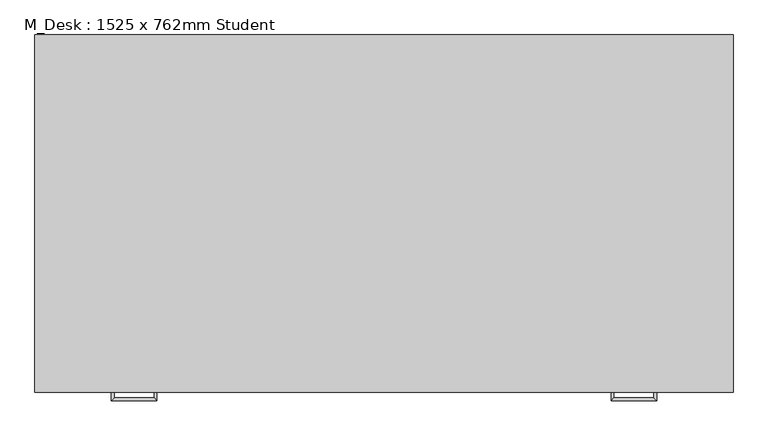
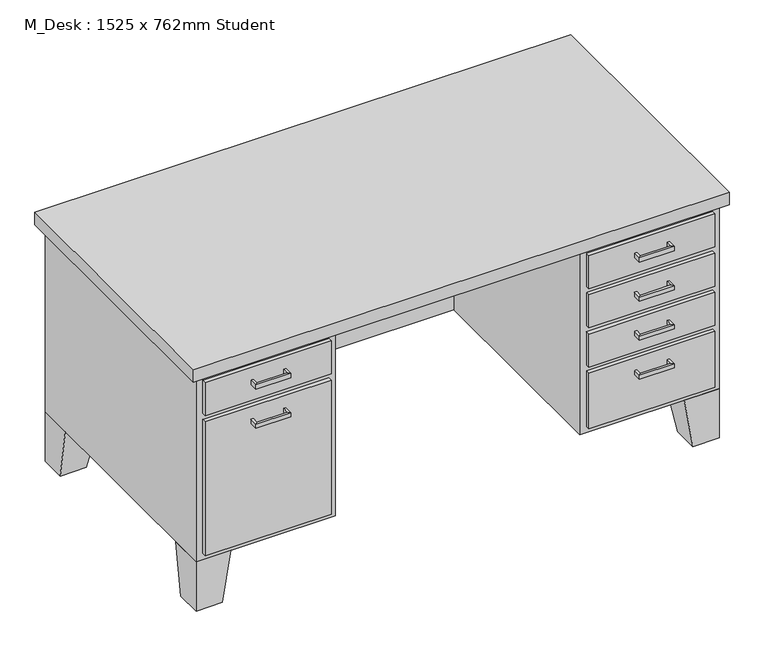
"""IFC4 building model written with IfcOpenShell, lengths in millimetres: furniture geometry, M_Desk : 1525 x 762mm Student."""

import ifcopenshell
import ifcopenshell.guid

model = None  # the IFC model being written
_history = None  # IfcOwnerHistory: only IFC2X3 demands one
_inside = {}  # id of a spatial element -> (the spatial element, [elements in it])
_under = {}  # id of a project, library or spatial element -> (it, [spatial elements below it])
_declared = {}  # id of a project -> (the project, [libraries it declares])
_typed = {}  # id of a type object -> (the type object, [elements of that type])
_made_of = {}  # id of a material, layer set ... -> (it, [elements and type objects made of it])


def new_model(schema):
    """Start an empty IFC model of exactly this schema.

    Asked for "IFC4X3", IfcOpenShell would pick the latest addendum, in which some entities
    have other attributes; the version numbers below select the first issue.
    IFC2X3 requires an IfcOwnerHistory on every rooted entity: one is made here for all.
    """
    global model, _history
    if schema == "IFC4X3":
        model = ifcopenshell.file(schema_version=(4, 3, 0, 0))
    else:
        model = ifcopenshell.file(schema=schema)
    _inside.clear()
    _under.clear()
    _declared.clear()
    _typed.clear()
    _made_of.clear()
    _history = None
    if model.schema == "IFC2X3":
        org = make("IfcOrganization", Name="unknown")
        user = make(
            "IfcPersonAndOrganization",
            ThePerson=make("IfcPerson", FamilyName="unknown"),
            TheOrganization=org,
        )
        app = make(
            "IfcApplication",
            ApplicationDeveloper=org,
            Version="unknown",
            ApplicationFullName="unknown",
            ApplicationIdentifier="unknown",
        )
        _history = make(
            "IfcOwnerHistory",
            OwningUser=user,
            OwningApplication=app,
            ChangeAction="ADDED",
            CreationDate=0,
        )
    return model


def make(cls, **values):
    """One entity of the class cls with the attributes given. An attribute that is None is left unset."""
    return model.create_entity(
        cls, **{name: value for name, value in values.items() if value is not None}
    )


def rooted(cls, **values):
    """An entity with a GlobalId (a new one), such as an element, a storey or a relation."""
    return make(cls, GlobalId=ifcopenshell.guid.new(), OwnerHistory=_history, **values)


def si_unit(unit_type, name, prefix=None):
    """IfcSIUnit, for example si_unit("LENGTHUNIT", "METRE", prefix="MILLI")."""
    return make("IfcSIUnit", UnitType=unit_type, Prefix=prefix, Name=name)


def assignment(units):
    """IfcUnitAssignment: the units of a project."""
    return None if units is None else make("IfcUnitAssignment", Units=units)


def point(xyz):
    """IfcCartesianPoint."""
    return None if xyz is None else make("IfcCartesianPoint", Coordinates=xyz)


def direction(xyz):
    """IfcDirection."""
    return None if xyz is None else make("IfcDirection", DirectionRatios=xyz)


def frame(location, z_axis=None, x_axis=None):
    """IfcAxis2Placement3D, a coordinate frame: its origin and axes. An axis left out is left unset."""
    return make(
        "IfcAxis2Placement3D",
        Location=point(location),
        Axis=direction(z_axis),
        RefDirection=direction(x_axis),
    )


def origin():
    """The frame at (0, 0, 0) with its axes left unset."""
    return frame((0.0, 0.0, 0.0))


def place(relative_to, where):
    """IfcLocalPlacement: puts the frame where relative to a parent placement (None: the world)."""
    return make(
        "IfcLocalPlacement", PlacementRelTo=relative_to, RelativePlacement=where
    )


def context(
    kind, dimensions, precision=None, world=None, true_north=None, identifier=None
):
    """IfcGeometricRepresentationContext, for example the 3D "Model" context."""
    return make(
        "IfcGeometricRepresentationContext",
        ContextIdentifier=identifier,
        ContextType=kind,
        CoordinateSpaceDimension=dimensions,
        Precision=precision,
        WorldCoordinateSystem=world,
        TrueNorth=true_north,
    )


def project(units=None, contexts=None):
    """IfcProject with its units and contexts."""
    return rooted(
        "IfcProject",
        Name="project",
        RepresentationContexts=contexts,
        UnitsInContext=assignment(units),
    )


def spatial(cls, under=None, at=None, **own):
    """A site, building, storey or space (cls), placed at a placement, below another one or the project."""
    s = rooted(cls, ObjectPlacement=at, **own)
    if under is not None:
        _under.setdefault(under.id(), (under, []))[1].append(s)
    return s


def polyline(points):
    """IfcPolyline through the points."""
    return make("IfcPolyline", Points=[point(p) for p in points])


def outline(outer, holes=None, kind="AREA"):
    """IfcArbitraryClosedProfileDef: a profile drawn as a closed curve; with holes, ...WithVoids."""
    if holes is None:
        return make("IfcArbitraryClosedProfileDef", ProfileType=kind, OuterCurve=outer)
    return make(
        "IfcArbitraryProfileDefWithVoids",
        ProfileType=kind,
        OuterCurve=outer,
        InnerCurves=holes,
    )


def extrude(swept, where, along, depth):
    """IfcExtrudedAreaSolid: the profile swept, set in the frame where, extruded along a direction by depth."""
    return make(
        "IfcExtrudedAreaSolid",
        SweptArea=swept,
        Position=where,
        ExtrudedDirection=direction(along),
        Depth=depth,
    )


def faces_of(points, faces, orient=None, outer=None):
    """IfcFace entities. A face is a list of loops; a loop is a list of indices into points, from 0.

    orient and outer hold one flag for each loop. By default every Orientation is true, the
    first loop of a face is its IfcFaceOuterBound and the others are IfcFaceBound.
    """
    made = []
    for i, loops in enumerate(faces):
        bounds = []
        for j, loop in enumerate(loops):
            is_outer = j == 0 if outer is None else outer[i][j]
            bounds.append(
                make(
                    "IfcFaceOuterBound" if is_outer else "IfcFaceBound",
                    Bound=make("IfcPolyLoop", Polygon=[points[k] for k in loop]),
                    Orientation=True if orient is None else orient[i][j],
                )
            )
        made.append(make("IfcFace", Bounds=bounds))
    return made


def faceted_brep(points, faces, orient=None, outer=None, voids=None):
    """IfcFacetedBrep: a solid bounded by flat faces; with voids (closed shells), ...WithVoids."""
    shared = [point(p) for p in points]
    hull = make("IfcClosedShell", CfsFaces=faces_of(shared, faces, orient, outer))
    if voids is None:
        return make("IfcFacetedBrep", Outer=hull)
    return make(
        "IfcFacetedBrepWithVoids",
        Outer=hull,
        Voids=[
            make(cls, CfsFaces=faces_of(shared, fs, o, b)) for cls, fs, o, b in voids
        ],
    )


def shape(context_of_items, identifier, shape_type, items):
    """IfcShapeRepresentation: the items that make up one representation, for example the "Body"."""
    return make(
        "IfcShapeRepresentation",
        ContextOfItems=context_of_items,
        RepresentationIdentifier=identifier,
        RepresentationType=shape_type,
        Items=items,
    )


def source(mapping_origin, context_of_items, identifier, shape_type, items):
    """IfcRepresentationMap: a shape defined once, which mapped items show again and again."""
    return make(
        "IfcRepresentationMap",
        MappingOrigin=mapping_origin,
        MappedRepresentation=shape(context_of_items, identifier, shape_type, items),
    )


def transform(
    local_origin,
    x_axis=None,
    y_axis=None,
    z_axis=None,
    scale=None,
    scale2=None,
    scale3=None,
    uniform=True,
):
    """IfcCartesianTransformationOperator3D, or its non-uniform kind. x_axis, y_axis, z_axis: its Axis1, 2, 3."""
    if uniform:
        return make(
            "IfcCartesianTransformationOperator3D",
            Axis1=direction(x_axis),
            Axis2=direction(y_axis),
            LocalOrigin=point(local_origin),
            Scale=scale,
            Axis3=direction(z_axis),
        )
    return make(
        "IfcCartesianTransformationOperator3DnonUniform",
        Axis1=direction(x_axis),
        Axis2=direction(y_axis),
        LocalOrigin=point(local_origin),
        Scale=scale,
        Axis3=direction(z_axis),
        Scale2=scale2,
        Scale3=scale3,
    )


def mapped(mapping_source, mapping_target):
    """IfcMappedItem: shows the shape of a source again, moved by a transform."""
    return make(
        "IfcMappedItem", MappingSource=mapping_source, MappingTarget=mapping_target
    )


def made_of(thing, what):
    """Note that an element or type object is made of a material, layer set ...; save() writes the relation."""
    if what is not None:
        _made_of.setdefault(what.id(), (what, []))[1].append(thing)
    return thing


def element(
    cls,
    number,
    at=None,
    inside=None,
    cuts=None,
    type_object=None,
    material=None,
    context=None,
    identifier="Body",
    shape_type=None,
    held_by="IfcProductDefinitionShape",
    body=None,
    shapes=None,
    **own,
):
    """One element of the class cls, such as IfcWall. Its Tag is "e" and its number.

    at: its placement. inside: the storey or other place that contains it. cuts: it is an
    opening in that element (IfcRelVoidsElement). A single representation is given by context,
    identifier, shape_type and body (its items); several are given by shapes. held_by: the class
    of the entity that holds the representations. save() writes the other relations.
    """
    e = rooted(cls, Tag="e%d" % number, ObjectPlacement=at, **own)
    if body is not None:
        shapes = [shape(context, identifier, shape_type, body)]
    if shapes is not None:
        e.Representation = make(held_by, Representations=shapes)
    if inside is not None:
        _inside.setdefault(inside.id(), (inside, []))[1].append(e)
    if cuts is not None:
        rooted(
            "IfcRelVoidsElement", RelatingBuildingElement=cuts, RelatedOpeningElement=e
        )
    if type_object is not None:
        _typed.setdefault(type_object.id(), (type_object, []))[1].append(e)
    return made_of(e, material)


def aggregate(whole, parts):
    """IfcRelAggregates: a whole, such as a stair, and the parts it consists of."""
    return rooted("IfcRelAggregates", RelatingObject=whole, RelatedObjects=parts)


def save(model, path):
    """Write the relations noted so far, then the file.

    IfcRelAggregates (storeys below a building ...), IfcRelContainedInSpatialStructure (elements
    in a storey), IfcRelDefinesByType, IfcRelAssociatesMaterial and IfcRelDeclares: one each for
    every whole, place, type object, material and project.
    """
    for whole, parts in _under.values():
        aggregate(whole, parts)
    for where, things in _inside.values():
        rooted(
            "IfcRelContainedInSpatialStructure",
            RelatedElements=things,
            RelatingStructure=where,
        )
    for kind, things in _typed.values():
        rooted("IfcRelDefinesByType", RelatedObjects=things, RelatingType=kind)
    for what, things in _made_of.values():
        rooted("IfcRelAssociatesMaterial", RelatedObjects=things, RelatingMaterial=what)
    for by, libraries in _declared.values():
        rooted("IfcRelDeclares", RelatingContext=by, RelatedDefinitions=libraries)
    model.write(path)


def m_desk_1525_x_762mm_student_34485ced(model_context):
    return source(origin(), model_context, "Body", "SolidModel", [
        extrude(outline(polyline([(1118.1, 0.0), (1118.1, 635.0), (405.9, 635.0), (405.9, 0.0), (-0.5, 0.0), (-0.5, 762.0), (1524.5, 762.0), (1524.5, 0.0), (1118.1, 0.0)])), frame((0.0, 0.0, 152.0), z_axis=(0.0, 0.0, 1.0), x_axis=(1.0, 0.0, 0.0)), (0.0, 0.0, 1.0), 571.9),
        extrude(outline(polyline([(-19.55, -19.05), (-19.55, 781.05), (1543.55, 781.05), (1543.55, -19.05), (-19.55, -19.05)])), frame((0.0, 0.0, 723.9), z_axis=(0.0, 0.0, 1.0), x_axis=(1.0, 0.0, 0.0)), (0.0, 0.0, 1.0), 38.1),
        faceted_brep([(1422.9, 0.0, 152.0), (1524.5, 0.0, 152.0), (1524.5, 101.6, 152.0), (1422.9, 101.6, 152.0), (1448.3, 0.0, 0.0), (1448.3, 76.2, 0.0), (1524.5, 76.2, 0.0), (1524.5, 0.0, 0.0)], [[[0, 1, 2, 3]], [[4, 5, 6, 7]], [[4, 7, 1, 0]], [[7, 6, 2, 1]], [[6, 5, 3, 2]], [[5, 4, 0, 3]]]),
        faceted_brep([(1422.9, 762.0, 152.0), (1422.9, 660.4, 152.0), (1524.5, 660.4, 152.0), (1524.5, 762.0, 152.0), (1448.3, 762.0, 0.0), (1524.5, 762.0, 0.0), (1524.5, 685.8, 0.0), (1448.3, 685.8, 0.0)], [[[0, 1, 2, 3]], [[4, 5, 6, 7]], [[4, 7, 1, 0]], [[7, 6, 2, 1]], [[6, 5, 3, 2]], [[5, 4, 0, 3]]]),
        faceted_brep([(101.1, 762.0, 152.0), (-0.5, 762.0, 152.0), (-0.5, 660.4, 152.0), (101.1, 660.4, 152.0), (75.7, 762.0, 0.0), (75.7, 685.8, 0.0), (-0.5, 685.8, 0.0), (-0.5, 762.0, 0.0)], [[[0, 1, 2, 3]], [[4, 5, 6, 7]], [[4, 7, 1, 0]], [[7, 6, 2, 1]], [[6, 5, 3, 2]], [[5, 4, 0, 3]]]),
        faceted_brep([(101.1, 0.0, 152.0), (101.1, 101.6, 152.0), (-0.5, 101.6, 152.0), (-0.5, 0.0, 152.0), (75.7, 0.0, 0.0), (-0.5, 0.0, 0.0), (-0.5, 76.2, 0.0), (75.7, 76.2, 0.0)], [[[0, 1, 2, 3]], [[4, 5, 6, 7]], [[4, 7, 1, 0]], [[7, 6, 2, 1]], [[6, 5, 3, 2]], [[5, 4, 0, 3]]]),
        extrude(outline(polyline([(1137.15, 0.0), (1505.45, 0.0), (1505.45, -12.7), (1137.15, -12.7), (1137.15, 0.0)])), frame((0.0, 0.0, 602.85), z_axis=(0.0, 0.0, 1.0), x_axis=(1.0, 0.0, 0.0)), (0.0, 0.0, 1.0), 102.0),
        extrude(outline(polyline([(1137.15, 0.0), (1505.45, 0.0), (1505.45, -12.7), (1137.15, -12.7), (1137.15, 0.0)])), frame((0.0, 0.0, 171.05), z_axis=(0.0, 0.0, 1.0), x_axis=(1.0, 0.0, 0.0)), (0.0, 0.0, 1.0), 171.45),
        extrude(outline(polyline([(1137.15, 0.0), (1505.45, 0.0), (1505.45, -12.7), (1137.15, -12.7), (1137.15, 0.0)])), frame((0.0, 0.0, 482.2), z_axis=(0.0, 0.0, 1.0), x_axis=(1.0, 0.0, 0.0)), (0.0, 0.0, 1.0), 101.6),
        extrude(outline(polyline([(1137.15, 0.0), (1505.45, 0.0), (1505.45, -12.7), (1137.15, -12.7), (1137.15, 0.0)])), frame((0.0, 0.0, 361.55), z_axis=(0.0, 0.0, 1.0), x_axis=(1.0, 0.0, 0.0)), (0.0, 0.0, 1.0), 101.6),
        extrude(outline(polyline([(18.55, 0.0), (386.85, 0.0), (386.85, -12.7), (18.55, -12.7), (18.55, 0.0)])), frame((0.0, 0.0, 603.25), z_axis=(0.0, 0.0, 1.0), x_axis=(1.0, 0.0, 0.0)), (0.0, 0.0, 1.0), 101.6),
        extrude(outline(polyline([(18.55, 0.0), (386.85, 0.0), (386.85, -12.7), (18.55, -12.7), (18.55, 0.0)])), frame((0.0, 0.0, 171.05), z_axis=(0.0, 0.0, 1.0), x_axis=(1.0, 0.0, 0.0)), (0.0, 0.0, 1.0), 413.15),
        faceted_brep([(1365.75, -12.7, 304.8), (1372.1, -12.7, 304.8), (1372.1, -12.7, 292.1), (1365.75, -12.7, 292.1), (1365.75, -31.75, 304.8), (1372.1, -38.1, 304.8), (1372.1, -38.1, 292.1), (1365.75, -31.75, 292.1), (1276.85, -31.75, 304.8), (1270.5, -38.1, 304.8), (1270.5, -38.1, 292.1), (1276.85, -31.75, 292.1), (1276.85, -12.7, 304.8), (1276.85, -12.7, 292.1), (1270.5, -12.7, 292.1), (1270.5, -12.7, 304.8)], [[[0, 1, 2, 3]], [[1, 0, 4, 5]], [[2, 1, 5, 6]], [[3, 2, 6, 7]], [[0, 3, 7, 4]], [[5, 4, 8, 9]], [[6, 5, 9, 10]], [[7, 6, 10, 11]], [[4, 7, 11, 8]], [[12, 13, 14, 15]], [[9, 8, 12, 15]], [[10, 9, 15, 14]], [[11, 10, 14, 13]], [[8, 11, 13, 12]]]),
        faceted_brep([(1365.75, -12.7, 425.45), (1372.1, -12.7, 425.45), (1372.1, -12.7, 412.75), (1365.75, -12.7, 412.75), (1365.75, -31.75, 425.45), (1372.1, -38.1, 425.45), (1372.1, -38.1, 412.75), (1365.75, -31.75, 412.75), (1276.85, -31.75, 425.45), (1270.5, -38.1, 425.45), (1270.5, -38.1, 412.75), (1276.85, -31.75, 412.75), (1276.85, -12.7, 425.45), (1276.85, -12.7, 412.75), (1270.5, -12.7, 412.75), (1270.5, -12.7, 425.45)], [[[0, 1, 2, 3]], [[1, 0, 4, 5]], [[2, 1, 5, 6]], [[3, 2, 6, 7]], [[0, 3, 7, 4]], [[5, 4, 8, 9]], [[6, 5, 9, 10]], [[7, 6, 10, 11]], [[4, 7, 11, 8]], [[12, 13, 14, 15]], [[9, 8, 12, 15]], [[10, 9, 15, 14]], [[11, 10, 14, 13]], [[8, 11, 13, 12]]]),
        faceted_brep([(1365.75, -12.7, 546.1), (1372.1, -12.7, 546.1), (1372.1, -12.7, 533.4), (1365.75, -12.7, 533.4), (1365.75, -31.75, 546.1), (1372.1, -38.1, 546.1), (1372.1, -38.1, 533.4), (1365.75, -31.75, 533.4), (1276.85, -31.75, 546.1), (1270.5, -38.1, 546.1), (1270.5, -38.1, 533.4), (1276.85, -31.75, 533.4), (1276.85, -12.7, 546.1), (1276.85, -12.7, 533.4), (1270.5, -12.7, 533.4), (1270.5, -12.7, 546.1)], [[[0, 1, 2, 3]], [[1, 0, 4, 5]], [[2, 1, 5, 6]], [[3, 2, 6, 7]], [[0, 3, 7, 4]], [[5, 4, 8, 9]], [[6, 5, 9, 10]], [[7, 6, 10, 11]], [[4, 7, 11, 8]], [[12, 13, 14, 15]], [[9, 8, 12, 15]], [[10, 9, 15, 14]], [[11, 10, 14, 13]], [[8, 11, 13, 12]]]),
        faceted_brep([(1365.75, -12.7, 666.75), (1372.1, -12.7, 666.75), (1372.1, -12.7, 654.05), (1365.75, -12.7, 654.05), (1365.75, -31.75, 666.75), (1372.1, -38.1, 666.75), (1372.1, -38.1, 654.05), (1365.75, -31.75, 654.05), (1276.85, -31.75, 666.75), (1270.5, -38.1, 666.75), (1270.5, -38.1, 654.05), (1276.85, -31.75, 654.05), (1276.85, -12.7, 666.75), (1276.85, -12.7, 654.05), (1270.5, -12.7, 654.05), (1270.5, -12.7, 666.75)], [[[0, 1, 2, 3]], [[1, 0, 4, 5]], [[2, 1, 5, 6]], [[3, 2, 6, 7]], [[0, 3, 7, 4]], [[5, 4, 8, 9]], [[6, 5, 9, 10]], [[7, 6, 10, 11]], [[4, 7, 11, 8]], [[12, 13, 14, 15]], [[9, 8, 12, 15]], [[10, 9, 15, 14]], [[11, 10, 14, 13]], [[8, 11, 13, 12]]]),
        faceted_brep([(158.25, -12.7, 546.1), (158.25, -12.7, 533.4), (151.9, -12.7, 533.4), (151.9, -12.7, 546.1), (158.25, -31.75, 546.1), (158.25, -31.75, 533.4), (151.9, -38.1, 533.4), (151.9, -38.1, 546.1), (247.15, -31.75, 546.1), (247.15, -31.75, 533.4), (253.5, -38.1, 533.4), (253.5, -38.1, 546.1), (247.15, -12.7, 546.1), (253.5, -12.7, 546.1), (253.5, -12.7, 533.4), (247.15, -12.7, 533.4)], [[[0, 1, 2, 3]], [[1, 0, 4, 5]], [[2, 1, 5, 6]], [[3, 2, 6, 7]], [[0, 3, 7, 4]], [[5, 4, 8, 9]], [[6, 5, 9, 10]], [[7, 6, 10, 11]], [[4, 7, 11, 8]], [[12, 13, 14, 15]], [[9, 8, 12, 15]], [[10, 9, 15, 14]], [[11, 10, 14, 13]], [[8, 11, 13, 12]]]),
        faceted_brep([(158.25, -12.7, 666.75), (158.25, -12.7, 654.05), (151.9, -12.7, 654.05), (151.9, -12.7, 666.75), (158.25, -31.75, 666.75), (158.25, -31.75, 654.05), (151.9, -38.1, 654.05), (151.9, -38.1, 666.75), (247.15, -31.75, 666.75), (247.15, -31.75, 654.05), (253.5, -38.1, 654.05), (253.5, -38.1, 666.75), (247.15, -12.7, 666.75), (253.5, -12.7, 666.75), (253.5, -12.7, 654.05), (247.15, -12.7, 654.05)], [[[0, 1, 2, 3]], [[1, 0, 4, 5]], [[2, 1, 5, 6]], [[3, 2, 6, 7]], [[0, 3, 7, 4]], [[5, 4, 8, 9]], [[6, 5, 9, 10]], [[7, 6, 10, 11]], [[4, 7, 11, 8]], [[12, 13, 14, 15]], [[9, 8, 12, 15]], [[10, 9, 15, 14]], [[11, 10, 14, 13]], [[8, 11, 13, 12]]]),
    ])


if __name__ == "__main__":
    model = new_model("IFC4")
    model_context = context("Model", 3, world=origin())
    ifc_project = project(units=[si_unit("LENGTHUNIT", "METRE", prefix="MILLI")], contexts=[model_context])
    site = spatial("IfcSite", under=ifc_project)
    building = spatial("IfcBuilding", under=site)
    placement = place(None, origin())
    m_desk_1525_x_762mm_student_shape = m_desk_1525_x_762mm_student_34485ced(model_context)
    element("IfcFurniture", 1, ObjectType="M_Desk : 1525 x 762mm Student", at=placement, inside=building, context=model_context, shape_type="MappedRepresentation", body=[
        mapped(m_desk_1525_x_762mm_student_shape, transform((0.0, 0.0, 0.0), x_axis=(1.0, 0.0, 0.0), y_axis=(0.0, 1.0, 0.0), z_axis=(0.0, 0.0, 1.0))),
    ])
    save(model, "model.ifc")

# Revit data of these elements
# Type "M_Desk : 1525 x 762mm Student"
#   Depth = 762 mm
#   Height = 762 mm
#   Leg Height = 152 mm
#   Width = 1525 mm
#   Body Material = Laminate, Ivory, Matte
#   Handle/Leg Material = Steel, Chrome Plated
#   Top Material = Cherry
#   Default Elevation = 0
# Element 1 (IfcFurniture, "M_Desk : 1525 x 762mm Student")
#   Materials on its faces: "Steel, Chrome Plated", "Laminate, Ivory, Matte", "Cherry"
# Materials
#   "Laminate, Ivory, Matte": class "Plastic", colour RGB 244 244 244, transparency 0, Description = "Plastic Laminate - Ivory, Matte", Cost = 0
#   "Steel, Chrome Plated": class "Metal", colour RGB 17 17 17, transparency 0, Description = "Chromiuim plated steel", Cost = 0
#   "Cherry": class "Wood", colour RGB 158 77 40, transparency 0, Description = "Prunus Serotina", Cost = 0
